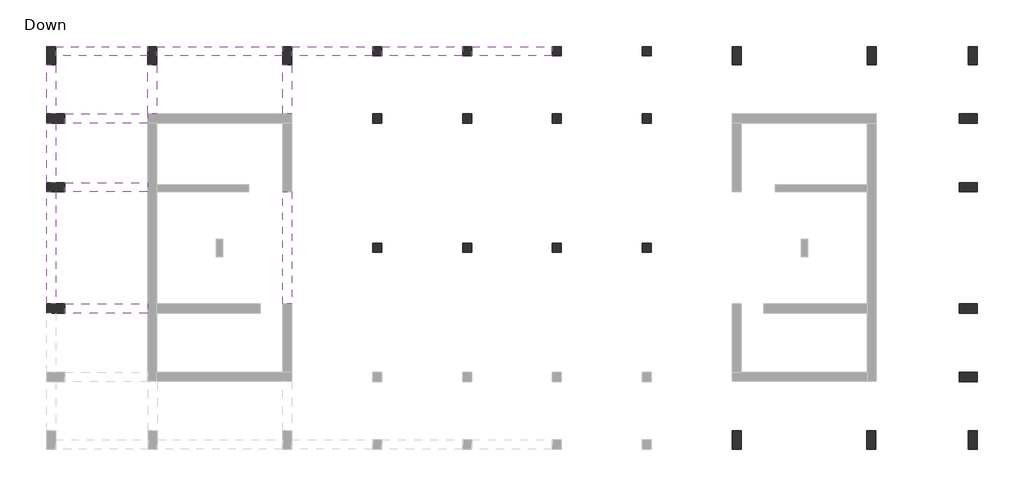
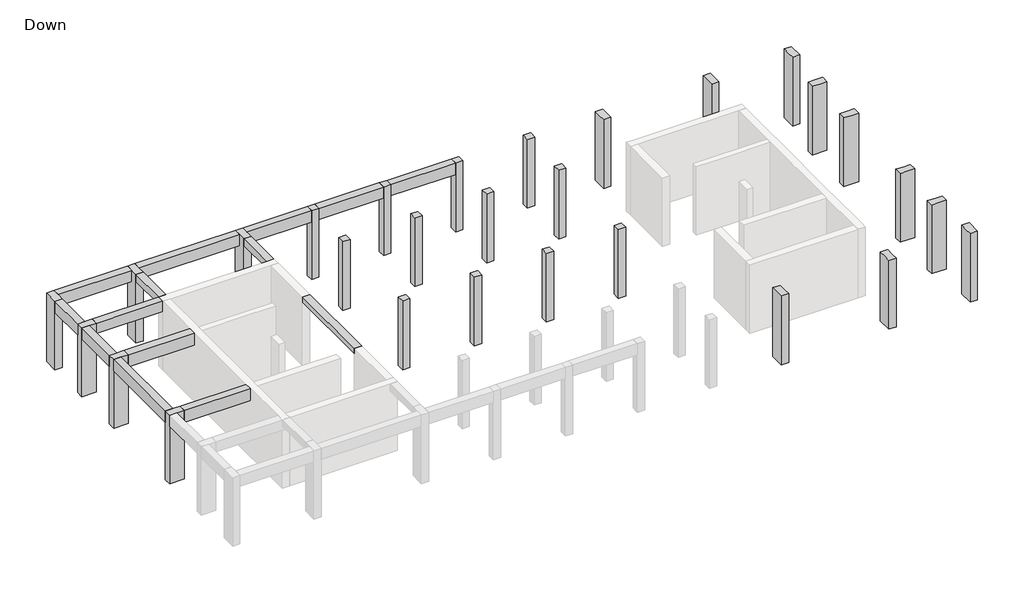
# One storey, part 2 of 2: 28 columns, 14 beams.
"""IFC4 building model written with IfcOpenShell, lengths in millimetres."""

from ifc_helpers import new_model, si_unit, frame, origin, place, context, project, spatial, polyline, outline, extrude, faceted_brep, element, save

model = new_model("IFC4")

# Units and contexts
model_context = context("Model", 3, world=origin())
ifc_project = project(units=[si_unit("LENGTHUNIT", "METRE", prefix="MILLI")], contexts=[model_context])

# Site, building, storey
site = spatial("IfcSite", under=ifc_project)
building = spatial("IfcBuilding", under=site)
storey = spatial("IfcBuildingStorey", under=building, Name="Down", Elevation=0.0)

# Beams
placement = place(None, origin())
element("IfcBeam", 1, ObjectType="Concrete Rectengular Beam : 40/30", at=placement, inside=storey, context=model_context, shape_type="SweptSolid", body=[
    extrude(outline(polyline([(-9870.3374688, 5392.831899), (-9470.3374688, 5392.831899), (-9470.3374688, 443.9061014), (-9870.3374688, 443.9061014), (-9870.3374688, 5392.831899)])), frame((0.0, 0.0, 3700.0), z_axis=(0.0, 0.0, 1.0), x_axis=(1.0, 0.0, 0.0)), (0.0, 0.0, 1.0), 300.0),
])
element("IfcBeam", 2, ObjectType="Concrete Rectengular Beam : 40/40", at=placement, inside=storey, context=model_context, shape_type="Brep", body=[
    faceted_brep([(-15412.8227448, 10981.7889465, 4000.0), (-15812.8227448, 10981.7889465, 4000.0), (-15812.8227448, 8813.6899891, 4000.0), (-15412.8227448, 8813.6899891, 4000.0), (-15812.8227448, 10981.7889465, 3600.0), (-15812.8227448, 8813.6899891, 3600.0), (-15812.8227448, 8813.6899891, 3850.0), (-15412.8227448, 10981.7889465, 3600.0), (-15412.8227448, 8813.6899891, 3600.0), (-15412.8227448, 8813.6899891, 3850.0)], [[[0, 1, 2, 3]], [[1, 4, 5, 6, 2]], [[4, 7, 8, 5]], [[7, 0, 3, 9, 8]], [[1, 0, 7, 4]], [[3, 2, 6, 5, 8, 9]]]),
])
element("IfcBeam", 3, ObjectType="Concrete Rectengular Beam : 40/40", at=placement, inside=storey, context=model_context, shape_type="Brep", body=[
    faceted_brep([(-9470.3374688, 10981.7889465, 4000.0), (-9870.3374688, 10981.7889465, 4000.0), (-9870.3374688, 8813.6899891, 4000.0), (-9470.3374688, 8813.6899891, 4000.0), (-9870.3374688, 10981.7889465, 3600.0), (-9870.3374688, 8813.6899891, 3600.0), (-9870.3374688, 8813.6899891, 3850.0), (-9470.3374688, 10981.7889465, 3600.0), (-9470.3374688, 8813.6899891, 3600.0)], [[[0, 1, 2, 3]], [[1, 4, 5, 6, 2]], [[4, 7, 8, 5]], [[7, 0, 3, 8]], [[1, 0, 7, 4]], [[3, 2, 6, 5, 8]]]),
])
element("IfcBeam", 4, ObjectType="Concrete Rectengular Beam : 40/60", at=placement, inside=storey, context=model_context, shape_type="Brep", body=[
    faceted_brep([(-19471.2573041, 8813.6899891, 4000.0), (-19471.2573041, 8413.6899891, 4000.0), (-15812.8227448, 8413.6899891, 4000.0), (-15812.8227448, 8813.6899891, 4000.0), (-19471.2573041, 8413.6899891, 3400.0), (-15812.8227448, 8413.6899891, 3400.0), (-15812.8227448, 8413.6899891, 3850.0), (-19471.2573041, 8813.6899891, 3400.0), (-15812.8227448, 8813.6899891, 3400.0), (-15812.8227448, 8813.6899891, 3850.0)], [[[0, 1, 2, 3]], [[1, 4, 5, 6, 2]], [[4, 7, 8, 5]], [[7, 0, 3, 9, 8]], [[1, 0, 7, 4]], [[3, 2, 6, 5, 8, 9]]]),
])
element("IfcBeam", 5, ObjectType="Concrete Rectengular Beam : 40/65", at=placement, inside=storey, context=model_context, shape_type="Brep", body=[
    faceted_brep([(-19871.2573041, 11781.7889465, 4000.0), (-19871.2573041, 11381.7889465, 4000.0), (-15812.8227448, 11381.7889465, 4000.0), (-15812.8227448, 11781.7889465, 4000.0), (-19871.2573041, 11781.7889465, 3350.0), (-15812.8227448, 11781.7889465, 3350.0), (-19871.2573041, 11381.7889465, 3350.0), (-15812.8227448, 11381.7889465, 3350.0), (-19871.2573041, 11381.7889465, 3850.0), (-15812.8227448, 11381.7889465, 3850.0)], [[[0, 1, 2, 3]], [[4, 0, 3, 5]], [[6, 4, 5, 7]], [[1, 8, 6, 7, 9, 2]], [[1, 0, 4, 6, 8]], [[3, 2, 9, 7, 5]]]),
])
element("IfcBeam", 6, ObjectType="Concrete Rectengular Beam : 40/65", at=placement, inside=storey, context=model_context, shape_type="Brep", body=[
    faceted_brep([(-15412.8227448, 11781.7889465, 4000.0), (-15412.8227448, 11381.7889465, 4000.0), (-9870.3374688, 11381.7889465, 4000.0), (-9870.3374688, 11781.7889465, 4000.0), (-15412.8227448, 11381.7889465, 3850.0), (-15412.8227448, 11381.7889465, 3350.0), (-9870.3374688, 11381.7889465, 3350.0), (-9870.3374688, 11381.7889465, 3850.0), (-15412.8227448, 11781.7889465, 3350.0), (-9870.3374688, 11781.7889465, 3350.0)], [[[0, 1, 2, 3]], [[1, 4, 5, 6, 7, 2]], [[5, 8, 9, 6]], [[8, 0, 3, 9]], [[1, 0, 8, 5, 4]], [[3, 2, 7, 6, 9]]]),
])
element("IfcBeam", 7, ObjectType="Concrete Rectengular Beam : 40/65", at=placement, inside=storey, context=model_context, shape_type="Brep", body=[
    faceted_brep([(-9470.3374688, 11781.7889465, 4000.0), (-9470.3374688, 11381.7889465, 4000.0), (-5908.6814696, 11381.7889465, 4000.0), (-5908.6814696, 11781.7889465, 4000.0), (-9470.3374688, 11381.7889465, 3770.0), (-9470.3374688, 11381.7889465, 3350.0), (-5908.6814696, 11381.7889465, 3350.0), (-9470.3374688, 11781.7889465, 3350.0), (-5908.6814696, 11781.7889465, 3350.0)], [[[0, 1, 2, 3]], [[1, 4, 5, 6, 2]], [[5, 7, 8, 6]], [[7, 0, 3, 8]], [[1, 0, 7, 5, 4]], [[3, 2, 6, 8]]]),
])
element("IfcBeam", 8, ObjectType="Concrete Rectengular Beam : 40/65", at=placement, inside=storey, context=model_context, shape_type="SweptSolid", body=[
    extrude(outline(polyline([(-5508.6814696, 11381.7889465), (-5508.6814696, 11781.7889465), (-1947.0254312, 11781.7889465), (-1947.0254312, 11381.7889465), (-5508.6814696, 11381.7889465)])), frame((0.0, 0.0, 3350.0), z_axis=(0.0, 0.0, 1.0), x_axis=(1.0, 0.0, 0.0)), (0.0, 0.0, 1.0), 650.0),
])
element("IfcBeam", 9, ObjectType="Concrete Rectengular Beam : 40/65", at=placement, inside=storey, context=model_context, shape_type="Brep", body=[
    faceted_brep([(-19871.2573041, 10981.7889465, 4000.0), (-20271.2573041, 10981.7889465, 4000.0), (-20271.2573041, 8813.6899891, 4000.0), (-19871.2573041, 8813.6899891, 4000.0), (-20271.2573041, 10981.7889465, 3350.0), (-20271.2573041, 8813.6899891, 3350.0), (-19871.2573041, 10981.7889465, 3350.0), (-19871.2573041, 8813.6899891, 3350.0), (-19871.2573041, 8813.6899891, 3850.0)], [[[0, 1, 2, 3]], [[1, 4, 5, 2]], [[4, 6, 7, 5]], [[6, 0, 3, 8, 7]], [[1, 0, 6, 4]], [[3, 2, 5, 7, 8]]]),
])
element("IfcBeam", 10, ObjectType="Concrete Rectengular Beam : 40/65", at=placement, inside=storey, context=model_context, shape_type="Brep", body=[
    faceted_brep([(-19871.2573041, 8413.6899891, 4000.0), (-20271.2573041, 8413.6899891, 4000.0), (-20271.2573041, 5788.9969998, 4000.0), (-19871.2573041, 5788.9969998, 4000.0), (-20271.2573041, 8413.6899891, 3350.0), (-20271.2573041, 5788.9969998, 3350.0), (-19871.2573041, 8413.6899891, 3350.0), (-19871.2573041, 5788.9969998, 3350.0), (-19871.2573041, 8413.6899891, 3850.0), (-19871.2573041, 5788.9969998, 3850.0)], [[[0, 1, 2, 3]], [[1, 4, 5, 2]], [[4, 6, 7, 5]], [[6, 8, 0, 3, 9, 7]], [[1, 0, 8, 6, 4]], [[3, 2, 5, 7, 9]]]),
])
element("IfcBeam", 11, ObjectType="Concrete Rectengular Beam : 40/65", at=placement, inside=storey, context=model_context, shape_type="Brep", body=[
    faceted_brep([(-19871.2573041, 5388.9969998, 4000.0), (-20271.2573041, 5388.9969998, 4000.0), (-20271.2573041, 443.9061014, 4000.0), (-19871.2573041, 443.9061014, 4000.0), (-20271.2573041, 5388.9969998, 3350.0), (-20271.2573041, 443.9061014, 3350.0), (-19871.2573041, 5388.9969998, 3350.0), (-19871.2573041, 443.9061014, 3350.0), (-19871.2573041, 5388.9969998, 3850.0), (-19871.2573041, 443.9061014, 3850.0)], [[[0, 1, 2, 3]], [[1, 4, 5, 2]], [[4, 6, 7, 5]], [[6, 8, 0, 3, 9, 7]], [[1, 0, 8, 6, 4]], [[3, 2, 5, 7, 9]]]),
])
element("IfcBeam", 12, ObjectType="Concrete Rectengular Beam : 40/65", at=placement, inside=storey, context=model_context, shape_type="SweptSolid", body=[
    extrude(outline(polyline([(-1547.0254312, 11381.7889465), (-1547.0254312, 11781.7889465), (2010.7993238, 11781.7889465), (2010.7993238, 11381.7889465), (-1547.0254312, 11381.7889465)])), frame((0.0, 0.0, 3350.0), z_axis=(0.0, 0.0, 1.0), x_axis=(1.0, 0.0, 0.0)), (0.0, 0.0, 1.0), 650.0),
])
element("IfcBeam", 13, ObjectType="Concrete Rectengular Beam : 40/70", at=placement, inside=storey, context=model_context, shape_type="Brep", body=[
    faceted_brep([(-19471.2573041, 443.9061014, 4000.0), (-19471.2573041, 43.9061014, 4000.0), (-15812.8227448, 43.9061014, 4000.0), (-15812.8227448, 443.9061014, 4000.0), (-19471.2573041, 43.9061014, 3300.0), (-15812.8227448, 43.9061014, 3300.0), (-15812.8227448, 43.9061014, 3850.0), (-19471.2573041, 443.9061014, 3300.0), (-15812.8227448, 443.9061014, 3300.0), (-15812.8227448, 443.9061014, 3850.0)], [[[0, 1, 2, 3]], [[1, 4, 5, 6, 2]], [[4, 7, 8, 5]], [[7, 0, 3, 9, 8]], [[1, 0, 7, 4]], [[3, 2, 6, 5, 8, 9]]]),
])
element("IfcBeam", 14, ObjectType="Concrete Rectengular Beam : 40/70", at=placement, inside=storey, context=model_context, shape_type="Brep", body=[
    faceted_brep([(-19471.2573041, 5788.9969998, 4000.0), (-19471.2573041, 5388.9969998, 4000.0), (-15812.8227448, 5388.9969998, 4000.0), (-15812.8227448, 5788.9969998, 4000.0), (-19471.2573041, 5388.9969998, 3300.0), (-15812.8227448, 5388.9969998, 3300.0), (-15812.8227448, 5388.9969998, 3850.0), (-19471.2573041, 5788.9969998, 3300.0), (-15812.8227448, 5788.9969998, 3300.0), (-15812.8227448, 5788.9969998, 3850.0)], [[[0, 1, 2, 3]], [[1, 4, 5, 6, 2]], [[4, 7, 8, 5]], [[7, 0, 3, 9, 8]], [[1, 0, 7, 4]], [[3, 2, 6, 5, 8, 9]]]),
])

# Columns
element("IfcColumn", 15, ObjectType="Concrete Rectengular Column : 40/40", at=placement, inside=storey, context=model_context, shape_type="Brep", body=[
    faceted_brep([(-5508.6814696, 8813.6899891, 0.0), (-5508.6814696, 8413.6899891, 0.0), (-5908.6814696, 8413.6899891, 0.0), (-5908.6814696, 8813.6899891, 0.0), (-5508.6814696, 8813.6899891, 4000.0), (-5508.6814696, 8413.6899891, 4000.0), (-5508.6814696, 8413.6899891, 3770.0), (-5508.6814696, 8813.6899891, 3770.0), (-5908.6814696, 8413.6899891, 4000.0), (-5908.6814696, 8413.6899891, 3770.0), (-5908.6814696, 8813.6899891, 4000.0), (-5908.6814696, 8813.6899891, 3770.0)], [[[0, 1, 2, 3]], [[4, 5, 6, 1, 0, 7]], [[5, 8, 9, 2, 1, 6]], [[8, 10, 11, 3, 2, 9]], [[10, 4, 7, 0, 3, 11]], [[4, 10, 8, 5]]]),
])
element("IfcColumn", 16, ObjectType="Concrete Rectengular Column : 40/40", at=placement, inside=storey, context=model_context, shape_type="Brep", body=[
    faceted_brep([(-1547.0254312, 8813.6899891, 0.0), (-1547.0254312, 8413.6899891, 0.0), (-1947.0254312, 8413.6899891, 0.0), (-1947.0254312, 8813.6899891, 0.0), (-1547.0254312, 8813.6899891, 4000.0), (-1547.0254312, 8413.6899891, 4000.0), (-1547.0254312, 8413.6899891, 3770.0), (-1547.0254312, 8813.6899891, 3770.0), (-1947.0254312, 8413.6899891, 4000.0), (-1947.0254312, 8413.6899891, 3770.0), (-1947.0254312, 8813.6899891, 4000.0), (-1947.0254312, 8813.6899891, 3770.0)], [[[0, 1, 2, 3]], [[4, 5, 6, 1, 0, 7]], [[5, 8, 9, 2, 1, 6]], [[8, 10, 11, 3, 2, 9]], [[10, 4, 7, 0, 3, 11]], [[4, 10, 8, 5]]]),
])
element("IfcColumn", 17, ObjectType="Concrete Rectengular Column : 40/40", at=placement, inside=storey, context=model_context, shape_type="Brep", body=[
    faceted_brep([(-1547.0254312, 3116.4509414, 0.0), (-1547.0254312, 2716.4509414, 0.0), (-1947.0254312, 2716.4509414, 0.0), (-1947.0254312, 3116.4509414, 0.0), (-1547.0254312, 3116.4509414, 4000.0), (-1547.0254312, 2716.4509414, 4000.0), (-1547.0254312, 2716.4509414, 3770.0), (-1547.0254312, 3116.4509414, 3770.0), (-1947.0254312, 2716.4509414, 4000.0), (-1947.0254312, 2716.4509414, 3770.0), (-1947.0254312, 3116.4509414, 4000.0), (-1947.0254312, 3116.4509414, 3770.0)], [[[0, 1, 2, 3]], [[4, 5, 6, 1, 0, 7]], [[5, 8, 9, 2, 1, 6]], [[8, 10, 11, 3, 2, 9]], [[10, 4, 7, 0, 3, 11]], [[4, 10, 8, 5]]]),
])
element("IfcColumn", 18, ObjectType="Concrete Rectengular Column : 40/40", at=placement, inside=storey, context=model_context, shape_type="Brep", body=[
    faceted_brep([(-5508.6814696, 3116.4509414, 0.0), (-5508.6814696, 2716.4509414, 0.0), (-5908.6814696, 2716.4509414, 0.0), (-5908.6814696, 3116.4509414, 0.0), (-5508.6814696, 3116.4509414, 4000.0), (-5508.6814696, 2716.4509414, 4000.0), (-5508.6814696, 2716.4509414, 3770.0), (-5508.6814696, 3116.4509414, 3770.0), (-5908.6814696, 2716.4509414, 4000.0), (-5908.6814696, 2716.4509414, 3770.0), (-5908.6814696, 3116.4509414, 4000.0), (-5908.6814696, 3116.4509414, 3770.0)], [[[0, 1, 2, 3]], [[4, 5, 6, 1, 0, 7]], [[5, 8, 9, 2, 1, 6]], [[8, 10, 11, 3, 2, 9]], [[10, 4, 7, 0, 3, 11]], [[4, 10, 8, 5]]]),
])
element("IfcColumn", 19, ObjectType="Concrete Rectengular Column : 40/40", at=placement, inside=storey, context=model_context, shape_type="Brep", body=[
    faceted_brep([(-5508.6814696, 11781.7889465, 0.0), (-5508.6814696, 11381.7889465, 0.0), (-5908.6814696, 11381.7889465, 0.0), (-5908.6814696, 11781.7889465, 0.0), (-5508.6814696, 11781.7889465, 4000.0), (-5508.6814696, 11381.7889465, 4000.0), (-5508.6814696, 11381.7889465, 3350.0), (-5508.6814696, 11781.7889465, 3350.0), (-5908.6814696, 11381.7889465, 4000.0), (-5908.6814696, 11381.7889465, 3350.0), (-5908.6814696, 11781.7889465, 4000.0), (-5908.6814696, 11781.7889465, 3350.0)], [[[0, 1, 2, 3]], [[4, 5, 6, 1, 0, 7]], [[5, 8, 9, 2, 1, 6]], [[8, 10, 11, 3, 2, 9]], [[10, 4, 7, 0, 3, 11]], [[4, 10, 8, 5]]]),
])
element("IfcColumn", 20, ObjectType="Concrete Rectengular Column : 40/40", at=placement, inside=storey, context=model_context, shape_type="Brep", body=[
    faceted_brep([(-1547.0254312, 11781.7889465, 0.0), (-1547.0254312, 11381.7889465, 0.0), (-1947.0254312, 11381.7889465, 0.0), (-1947.0254312, 11781.7889465, 0.0), (-1547.0254312, 11781.7889465, 4000.0), (-1547.0254312, 11381.7889465, 4000.0), (-1947.0254312, 11381.7889465, 4000.0), (-1947.0254312, 11381.7889465, 3350.0), (-1947.0254312, 11781.7889465, 4000.0), (-1947.0254312, 11781.7889465, 3350.0)], [[[0, 1, 2, 3]], [[4, 5, 1, 0]], [[5, 6, 7, 2, 1]], [[6, 8, 9, 3, 2, 7]], [[8, 4, 0, 3, 9]], [[4, 8, 6, 5]]]),
])
element("IfcColumn", 21, ObjectType="Concrete Rectengular Column : 40/40", at=placement, inside=storey, context=model_context, shape_type="Brep", body=[
    faceted_brep([(5972.4553623, 8813.6899891, 0.0), (6372.4553623, 8813.6899891, 0.0), (6372.4553623, 8413.6899891, 0.0), (5972.4553623, 8413.6899891, 0.0), (5972.4553623, 8813.6899891, 4000.0), (5972.4553623, 8813.6899891, 3770.0), (5972.4553623, 8413.6899891, 3770.0), (5972.4553623, 8413.6899891, 4000.0), (6372.4553623, 8413.6899891, 3770.0), (6372.4553623, 8413.6899891, 4000.0), (6372.4553623, 8813.6899891, 3770.0), (6372.4553623, 8813.6899891, 4000.0)], [[[0, 1, 2, 3]], [[4, 5, 0, 3, 6, 7]], [[7, 6, 3, 2, 8, 9]], [[9, 8, 2, 1, 10, 11]], [[11, 10, 1, 0, 5, 4]], [[4, 7, 9, 11]]]),
])
element("IfcColumn", 22, ObjectType="Concrete Rectengular Column : 40/40", at=placement, inside=storey, context=model_context, shape_type="Brep", body=[
    faceted_brep([(2010.7993238, 8813.6899891, 0.0), (2410.7993238, 8813.6899891, 0.0), (2410.7993238, 8413.6899891, 0.0), (2010.7993238, 8413.6899891, 0.0), (2010.7993238, 8813.6899891, 4000.0), (2010.7993238, 8813.6899891, 3770.0), (2010.7993238, 8413.6899891, 3770.0), (2010.7993238, 8413.6899891, 4000.0), (2410.7993238, 8413.6899891, 3770.0), (2410.7993238, 8413.6899891, 4000.0), (2410.7993238, 8813.6899891, 3770.0), (2410.7993238, 8813.6899891, 4000.0)], [[[0, 1, 2, 3]], [[4, 5, 0, 3, 6, 7]], [[7, 6, 3, 2, 8, 9]], [[9, 8, 2, 1, 10, 11]], [[11, 10, 1, 0, 5, 4]], [[4, 7, 9, 11]]]),
])
element("IfcColumn", 23, ObjectType="Concrete Rectengular Column : 40/40", at=placement, inside=storey, context=model_context, shape_type="Brep", body=[
    faceted_brep([(2010.7993238, 3116.4509414, 0.0), (2410.7993238, 3116.4509414, 0.0), (2410.7993238, 2716.4509414, 0.0), (2010.7993238, 2716.4509414, 0.0), (2010.7993238, 3116.4509414, 4000.0), (2010.7993238, 3116.4509414, 3770.0), (2010.7993238, 2716.4509414, 3770.0), (2010.7993238, 2716.4509414, 4000.0), (2410.7993238, 2716.4509414, 3770.0), (2410.7993238, 2716.4509414, 4000.0), (2410.7993238, 3116.4509414, 3770.0), (2410.7993238, 3116.4509414, 4000.0)], [[[0, 1, 2, 3]], [[4, 5, 0, 3, 6, 7]], [[7, 6, 3, 2, 8, 9]], [[9, 8, 2, 1, 10, 11]], [[11, 10, 1, 0, 5, 4]], [[4, 7, 9, 11]]]),
])
element("IfcColumn", 24, ObjectType="Concrete Rectengular Column : 40/40", at=placement, inside=storey, context=model_context, shape_type="Brep", body=[
    faceted_brep([(5972.4553623, 3116.4509414, 0.0), (6372.4553623, 3116.4509414, 0.0), (6372.4553623, 2716.4509414, 0.0), (5972.4553623, 2716.4509414, 0.0), (5972.4553623, 3116.4509414, 4000.0), (5972.4553623, 3116.4509414, 3770.0), (5972.4553623, 2716.4509414, 3770.0), (5972.4553623, 2716.4509414, 4000.0), (6372.4553623, 2716.4509414, 3770.0), (6372.4553623, 2716.4509414, 4000.0), (6372.4553623, 3116.4509414, 3770.0), (6372.4553623, 3116.4509414, 4000.0)], [[[0, 1, 2, 3]], [[4, 5, 0, 3, 6, 7]], [[7, 6, 3, 2, 8, 9]], [[9, 8, 2, 1, 10, 11]], [[11, 10, 1, 0, 5, 4]], [[4, 7, 9, 11]]]),
])
element("IfcColumn", 25, ObjectType="Concrete Rectengular Column : 40/40", at=placement, inside=storey, context=model_context, shape_type="Brep", body=[
    faceted_brep([(5972.4553623, 11781.7889465, 0.0), (6372.4553623, 11781.7889465, 0.0), (6372.4553623, 11381.7889465, 0.0), (5972.4553623, 11381.7889465, 0.0), (5972.4553623, 11781.7889465, 4000.0), (5972.4553623, 11781.7889465, 3350.0), (5972.4553623, 11381.7889465, 3350.0), (5972.4553623, 11381.7889465, 4000.0), (6372.4553623, 11381.7889465, 3350.0), (6372.4553623, 11381.7889465, 4000.0), (6372.4553623, 11781.7889465, 3350.0), (6372.4553623, 11781.7889465, 4000.0)], [[[0, 1, 2, 3]], [[4, 5, 0, 3, 6, 7]], [[7, 6, 3, 2, 8, 9]], [[9, 8, 2, 1, 10, 11]], [[11, 10, 1, 0, 5, 4]], [[4, 7, 9, 11]]]),
])
element("IfcColumn", 26, ObjectType="Concrete Rectengular Column : 40/40", at=placement, inside=storey, context=model_context, shape_type="Brep", body=[
    faceted_brep([(2010.7993238, 11781.7889465, 0.0), (2410.7993238, 11781.7889465, 0.0), (2410.7993238, 11381.7889465, 0.0), (2010.7993238, 11381.7889465, 0.0), (2010.7993238, 11781.7889465, 4000.0), (2010.7993238, 11381.7889465, 4000.0), (2410.7993238, 11381.7889465, 3350.0), (2410.7993238, 11381.7889465, 4000.0), (2410.7993238, 11781.7889465, 3350.0), (2410.7993238, 11781.7889465, 4000.0)], [[[0, 1, 2, 3]], [[4, 0, 3, 5]], [[5, 3, 2, 6, 7]], [[7, 6, 2, 1, 8, 9]], [[9, 8, 1, 0, 4]], [[4, 5, 7, 9]]]),
])
element("IfcColumn", 27, ObjectType="Concrete Rectengular Column : 40/80", at=placement, inside=storey, context=model_context, shape_type="Brep", body=[
    faceted_brep([(-19871.2573041, 11781.7889465, 0.0), (-19871.2573041, 10981.7889465, 0.0), (-20271.2573041, 10981.7889465, 0.0), (-20271.2573041, 11781.7889465, 0.0), (-19871.2573041, 11781.7889465, 4000.0), (-19871.2573041, 11381.7889465, 4000.0), (-19871.2573041, 10981.7889465, 4000.0), (-20271.2573041, 10981.7889465, 4000.0), (-20271.2573041, 11781.7889465, 4000.0)], [[[0, 1, 2, 3]], [[4, 5, 6, 1, 0]], [[6, 7, 2, 1]], [[7, 8, 3, 2]], [[8, 4, 0, 3]], [[4, 8, 7, 6, 5]]]),
])
element("IfcColumn", 28, ObjectType="Concrete Rectengular Column : 40/80", at=placement, inside=storey, context=model_context, shape_type="Brep", body=[
    faceted_brep([(-20271.2573041, 8813.6899891, 0.0), (-19471.2573041, 8813.6899891, 0.0), (-19471.2573041, 8413.6899891, 0.0), (-20271.2573041, 8413.6899891, 0.0), (-20271.2573041, 8813.6899891, 4000.0), (-19871.2573041, 8813.6899891, 4000.0), (-19471.2573041, 8813.6899891, 4000.0), (-19471.2573041, 8413.6899891, 4000.0), (-19871.2573041, 8413.6899891, 4000.0), (-20271.2573041, 8413.6899891, 4000.0)], [[[0, 1, 2, 3]], [[4, 5, 6, 1, 0]], [[6, 7, 2, 1]], [[7, 8, 9, 3, 2]], [[9, 4, 0, 3]], [[4, 9, 8, 7, 6, 5]]]),
])
element("IfcColumn", 29, ObjectType="Concrete Rectengular Column : 40/80", at=placement, inside=storey, context=model_context, shape_type="Brep", body=[
    faceted_brep([(-20271.2573041, 5788.9969998, 0.0), (-19471.2573041, 5788.9969998, 0.0), (-19471.2573041, 5388.9969998, 0.0), (-20271.2573041, 5388.9969998, 0.0), (-20271.2573041, 5788.9969998, 4000.0), (-19871.2573041, 5788.9969998, 4000.0), (-19471.2573041, 5788.9969998, 4000.0), (-19471.2573041, 5388.9969998, 4000.0), (-19871.2573041, 5388.9969998, 4000.0), (-20271.2573041, 5388.9969998, 4000.0)], [[[0, 1, 2, 3]], [[4, 5, 6, 1, 0]], [[6, 7, 2, 1]], [[7, 8, 9, 3, 2]], [[9, 4, 0, 3]], [[4, 9, 8, 7, 6, 5]]]),
])
element("IfcColumn", 30, ObjectType="Concrete Rectengular Column : 40/80", at=placement, inside=storey, context=model_context, shape_type="Brep", body=[
    faceted_brep([(-20271.2573041, 443.9061014, 0.0), (-19471.2573041, 443.9061014, 0.0), (-19471.2573041, 43.9061014, 0.0), (-20271.2573041, 43.9061014, 0.0), (-20271.2573041, 443.9061014, 4000.0), (-19871.2573041, 443.9061014, 4000.0), (-19471.2573041, 443.9061014, 4000.0), (-19471.2573041, 43.9061014, 4000.0), (-19871.2573041, 43.9061014, 4000.0), (-20271.2573041, 43.9061014, 4000.0)], [[[0, 1, 2, 3]], [[4, 5, 6, 1, 0]], [[6, 7, 2, 1]], [[7, 8, 9, 3, 2]], [[9, 4, 0, 3]], [[4, 9, 8, 7, 6, 5]]]),
])
element("IfcColumn", 31, ObjectType="Concrete Rectengular Column : 40/80", at=placement, inside=storey, context=model_context, shape_type="Brep", body=[
    faceted_brep([(-15412.8227448, 11781.7889465, 0.0), (-15412.8227448, 10981.7889465, 0.0), (-15812.8227448, 10981.7889465, 0.0), (-15812.8227448, 11781.7889465, 0.0), (-15412.8227448, 11781.7889465, 4000.0), (-15412.8227448, 11381.7889465, 4000.0), (-15412.8227448, 10981.7889465, 4000.0), (-15812.8227448, 10981.7889465, 4000.0), (-15812.8227448, 11381.7889465, 4000.0), (-15812.8227448, 11781.7889465, 4000.0)], [[[0, 1, 2, 3]], [[4, 5, 6, 1, 0]], [[6, 7, 2, 1]], [[7, 8, 9, 3, 2]], [[9, 4, 0, 3]], [[4, 9, 8, 7, 6, 5]]]),
])
element("IfcColumn", 32, ObjectType="Concrete Rectengular Column : 40/80", at=placement, inside=storey, context=model_context, shape_type="Brep", body=[
    faceted_brep([(-9470.3374688, 11781.7889465, 0.0), (-9470.3374688, 10981.7889465, 0.0), (-9870.3374688, 10981.7889465, 0.0), (-9870.3374688, 11781.7889465, 0.0), (-9470.3374688, 11781.7889465, 4000.0), (-9470.3374688, 11381.7889465, 4000.0), (-9470.3374688, 10981.7889465, 4000.0), (-9870.3374688, 10981.7889465, 4000.0), (-9870.3374688, 11381.7889465, 4000.0), (-9870.3374688, 11781.7889465, 4000.0)], [[[0, 1, 2, 3]], [[4, 5, 6, 1, 0]], [[6, 7, 2, 1]], [[7, 8, 9, 3, 2]], [[9, 4, 0, 3]], [[4, 9, 8, 7, 6, 5]]]),
])
element("IfcColumn", 33, ObjectType="Concrete Rectengular Column : 40/80", at=placement, inside=storey, context=model_context, shape_type="Brep", body=[
    faceted_brep([(20335.0311968, 11781.7889465, 0.0), (20735.0311968, 11781.7889465, 0.0), (20735.0311968, 10981.7889465, 0.0), (20335.0311968, 10981.7889465, 0.0), (20335.0311968, 11781.7889465, 4000.0), (20335.0311968, 10981.7889465, 4000.0), (20335.0311968, 11381.7889465, 4000.0), (20735.0311968, 10981.7889465, 4000.0), (20735.0311968, 11781.7889465, 4000.0)], [[[0, 1, 2, 3]], [[4, 0, 3, 5, 6]], [[5, 3, 2, 7]], [[7, 2, 1, 8]], [[8, 1, 0, 4]], [[4, 6, 5, 7, 8]]]),
])
element("IfcColumn", 34, ObjectType="Concrete Rectengular Column : 40/80", at=placement, inside=storey, context=model_context, shape_type="Brep", body=[
    faceted_brep([(20735.0311968, 8813.6899891, 0.0), (20735.0311968, 8413.6899891, 0.0), (19935.0311968, 8413.6899891, 0.0), (19935.0311968, 8813.6899891, 0.0), (20735.0311968, 8813.6899891, 4000.0), (19935.0311968, 8813.6899891, 4000.0), (20335.0311968, 8813.6899891, 4000.0), (19935.0311968, 8413.6899891, 4000.0), (20735.0311968, 8413.6899891, 4000.0), (20335.0311968, 8413.6899891, 4000.0)], [[[0, 1, 2, 3]], [[4, 0, 3, 5, 6]], [[5, 3, 2, 7]], [[7, 2, 1, 8, 9]], [[8, 1, 0, 4]], [[4, 6, 5, 7, 9, 8]]]),
])
element("IfcColumn", 35, ObjectType="Concrete Rectengular Column : 40/80", at=placement, inside=storey, context=model_context, shape_type="Brep", body=[
    faceted_brep([(20735.0311968, 5788.9969998, 0.0), (20735.0311968, 5388.9969998, 0.0), (19935.0311968, 5388.9969998, 0.0), (19935.0311968, 5788.9969998, 0.0), (20735.0311968, 5788.9969998, 4000.0), (19935.0311968, 5788.9969998, 4000.0), (20335.0311968, 5788.9969998, 4000.0), (19935.0311968, 5388.9969998, 4000.0), (20735.0311968, 5388.9969998, 4000.0), (20335.0311968, 5388.9969998, 4000.0)], [[[0, 1, 2, 3]], [[4, 0, 3, 5, 6]], [[5, 3, 2, 7]], [[7, 2, 1, 8, 9]], [[8, 1, 0, 4]], [[4, 6, 5, 7, 9, 8]]]),
])
element("IfcColumn", 36, ObjectType="Concrete Rectengular Column : 40/80", at=placement, inside=storey, context=model_context, shape_type="Brep", body=[
    faceted_brep([(20735.0311968, 443.9061014, 0.0), (20735.0311968, 43.9061014, 0.0), (19935.0311968, 43.9061014, 0.0), (19935.0311968, 443.9061014, 0.0), (20735.0311968, 443.9061014, 4000.0), (19935.0311968, 443.9061014, 4000.0), (20335.0311968, 443.9061014, 4000.0), (19935.0311968, 43.9061014, 4000.0), (20735.0311968, 43.9061014, 4000.0), (20335.0311968, 43.9061014, 4000.0)], [[[0, 1, 2, 3]], [[4, 0, 3, 5, 6]], [[5, 3, 2, 7]], [[7, 2, 1, 8, 9]], [[8, 1, 0, 4]], [[4, 6, 5, 7, 9, 8]]]),
])
element("IfcColumn", 37, ObjectType="Concrete Rectengular Column : 40/80", at=placement, inside=storey, context=model_context, shape_type="Brep", body=[
    faceted_brep([(20735.0311968, -2574.5007845, 0.0), (20735.0311968, -2974.5007845, 0.0), (19935.0311968, -2974.5007845, 0.0), (19935.0311968, -2574.5007845, 0.0), (20735.0311968, -2574.5007845, 4000.0), (19935.0311968, -2574.5007845, 4000.0), (20335.0311968, -2574.5007845, 4000.0), (19935.0311968, -2974.5007845, 4000.0), (20735.0311968, -2974.5007845, 4000.0), (20335.0311968, -2974.5007845, 4000.0)], [[[0, 1, 2, 3]], [[4, 0, 3, 5, 6]], [[5, 3, 2, 7]], [[7, 2, 1, 8, 9]], [[8, 1, 0, 4]], [[4, 6, 5, 7, 9, 8]]]),
])
element("IfcColumn", 38, ObjectType="Concrete Rectengular Column : 40/80", at=placement, inside=storey, context=model_context, shape_type="Brep", body=[
    faceted_brep([(20335.0311968, -5152.7195656, 0.0), (20735.0311968, -5152.7195656, 0.0), (20735.0311968, -5952.7195656, 0.0), (20335.0311968, -5952.7195656, 0.0), (20335.0311968, -5152.7195656, 4000.0), (20335.0311968, -5952.7195656, 4000.0), (20335.0311968, -5548.8870638, 4000.0), (20735.0311968, -5952.7195656, 4000.0), (20735.0311968, -5152.7195656, 4000.0)], [[[0, 1, 2, 3]], [[4, 0, 3, 5, 6]], [[5, 3, 2, 7]], [[7, 2, 1, 8]], [[8, 1, 0, 4]], [[4, 6, 5, 7, 8]]]),
])
element("IfcColumn", 39, ObjectType="Concrete Rectengular Column : 40/80", at=placement, inside=storey, context=model_context, shape_type="Brep", body=[
    faceted_brep([(15855.0311968, -5152.7195656, 0.0), (16255.0311968, -5152.7195656, 0.0), (16255.0311968, -5952.7195656, 0.0), (15855.0311968, -5952.7195656, 0.0), (15855.0311968, -5152.7195656, 4000.0), (15855.0311968, -5952.7195656, 4000.0), (15855.0311968, -5548.8870638, 4000.0), (16255.0311968, -5952.7195656, 4000.0), (16255.0311968, -5152.7195656, 4000.0), (16255.0311968, -5548.8870638, 4000.0)], [[[0, 1, 2, 3]], [[4, 0, 3, 5, 6]], [[5, 3, 2, 7]], [[7, 2, 1, 8, 9]], [[8, 1, 0, 4]], [[4, 6, 5, 7, 9, 8]]]),
])
element("IfcColumn", 40, ObjectType="Concrete Rectengular Column : 40/80", at=placement, inside=storey, context=model_context, shape_type="Brep", body=[
    faceted_brep([(9934.1113614, -5152.7195656, 0.0), (10334.1113614, -5152.7195656, 0.0), (10334.1113614, -5952.7195656, 0.0), (9934.1113614, -5952.7195656, 0.0), (9934.1113614, -5152.7195656, 4000.0), (9934.1113614, -5952.7195656, 4000.0), (9934.1113614, -5548.8870638, 4000.0), (10334.1113614, -5952.7195656, 4000.0), (10334.1113614, -5152.7195656, 4000.0), (10334.1113614, -5548.8870638, 4000.0)], [[[0, 1, 2, 3]], [[4, 0, 3, 5, 6]], [[5, 3, 2, 7]], [[7, 2, 1, 8, 9]], [[8, 1, 0, 4]], [[4, 6, 5, 7, 9, 8]]]),
])
element("IfcColumn", 41, ObjectType="Concrete Rectengular Column : 40/80", at=placement, inside=storey, context=model_context, shape_type="Brep", body=[
    faceted_brep([(15876.5966375, 11781.7889465, 0.0), (16276.5966375, 11781.7889465, 0.0), (16276.5966375, 10981.7889465, 0.0), (15876.5966375, 10981.7889465, 0.0), (15876.5966375, 11781.7889465, 4000.0), (15876.5966375, 10981.7889465, 4000.0), (15876.5966375, 11381.7889465, 4000.0), (16276.5966375, 10981.7889465, 4000.0), (16276.5966375, 11781.7889465, 4000.0), (16276.5966375, 11381.7889465, 4000.0)], [[[0, 1, 2, 3]], [[4, 0, 3, 5, 6]], [[5, 3, 2, 7]], [[7, 2, 1, 8, 9]], [[8, 1, 0, 4]], [[4, 6, 5, 7, 9, 8]]]),
])
element("IfcColumn", 42, ObjectType="Concrete Rectengular Column : 40/80", at=placement, inside=storey, context=model_context, shape_type="Brep", body=[
    faceted_brep([(9934.1113614, 11781.7889465, 0.0), (10334.1113614, 11781.7889465, 0.0), (10334.1113614, 10981.7889465, 0.0), (9934.1113614, 10981.7889465, 0.0), (9934.1113614, 11781.7889465, 4000.0), (9934.1113614, 10981.7889465, 4000.0), (9934.1113614, 11381.7889465, 4000.0), (10334.1113614, 10981.7889465, 4000.0), (10334.1113614, 11781.7889465, 4000.0), (10334.1113614, 11381.7889465, 4000.0)], [[[0, 1, 2, 3]], [[4, 0, 3, 5, 6]], [[5, 3, 2, 7]], [[7, 2, 1, 8, 9]], [[8, 1, 0, 4]], [[4, 6, 5, 7, 9, 8]]]),
])

save(model, "model.ifc")

# Revit data of these elements
# Type "Concrete Rectengular Beam : 40/30"
#   Length [instance default] = 152.4 cm
#   b = 40 cm
#   h = 30 cm
#   Structural Material [instance default] = Concrete
#   Assembly Code = ""
# Type "Concrete Rectengular Beam : 40/40"
#   Length [instance default] = 152.4 cm
#   b = 40 cm
#   h = 40 cm
#   Structural Material [instance default] = Concrete
#   Assembly Code = ""
# Type "Concrete Rectengular Beam : 40/60"
#   Length [instance default] = 152.4 cm
#   b = 40 cm
#   h = 60 cm
#   Structural Material [instance default] = Concrete
#   Assembly Code = ""
# Type "Concrete Rectengular Beam : 40/65"
#   Length [instance default] = 152.4 cm
#   b = 40 cm
#   h = 65 cm
#   Structural Material [instance default] = Concrete
#   Assembly Code = ""
# Type "Concrete Rectengular Beam : 40/70"
#   Length [instance default] = 152.4 cm
#   b = 40 cm
#   h = 70 cm
#   Structural Material [instance default] = Concrete
#   Assembly Code = ""
# Type "Concrete Rectengular Column : 40/40"
#   b = 40 cm
#   h = 40 cm
#   Structural Material [instance default] = Concrete
# Type "Concrete Rectengular Column : 40/80"
#   b = 40 cm
#   h = 80 cm
#   Structural Material [instance default] = Concrete
# Element 1 (IfcBeam, "Concrete Rectengular Beam : 40/30")
#   Comments = ""
#   Mark = "B1"
#   SOFiSTiK_AMG_Comments = ""
#   SOFiSTiK_AMG_Scheduled = yes
#   SOFiSTiK_AMG_Adjusted = yes
#   Structural Material = Concrete
#   Phase Created = New Construction
#   Materials on its faces: "Concrete"
# Element 2 (IfcBeam, "Concrete Rectengular Beam : 40/40")
#   Comments = ""
#   Mark = "B5"
#   SOFiSTiK_AMG_Comments = ""
#   SOFiSTiK_AMG_Scheduled = yes
#   SOFiSTiK_AMG_Adjusted = yes
#   Structural Material = Concrete
#   Phase Created = New Construction
#   Materials on its faces: "Concrete"
# Element 3 (IfcBeam, "Concrete Rectengular Beam : 40/40")
#   Comments = ""
#   Mark = "B6"
#   SOFiSTiK_AMG_Comments = ""
#   SOFiSTiK_AMG_Scheduled = yes
#   SOFiSTiK_AMG_Adjusted = yes
#   Structural Material = Concrete
#   Phase Created = New Construction
#   Materials on its faces: "Concrete"
# Element 4 (IfcBeam, "Concrete Rectengular Beam : 40/60")
#   Comments = ""
#   Mark = "B11"
#   SOFiSTiK_AMG_Comments = ""
#   SOFiSTiK_AMG_Scheduled = yes
#   SOFiSTiK_AMG_Adjusted = yes
#   Structural Material = Concrete
#   Phase Created = New Construction
#   Materials on its faces: "Concrete"
# Element 5 (IfcBeam, "Concrete Rectengular Beam : 40/65")
#   Comments = ""
#   Mark = "B15"
#   SOFiSTiK_AMG_Comments = ""
#   SOFiSTiK_AMG_Scheduled = yes
#   SOFiSTiK_AMG_Adjusted = yes
#   Structural Material = Concrete
#   Phase Created = New Construction
#   Materials on its faces: "Concrete"
# Element 6 (IfcBeam, "Concrete Rectengular Beam : 40/65")
#   Comments = ""
#   Mark = "B16"
#   SOFiSTiK_AMG_Comments = ""
#   SOFiSTiK_AMG_Scheduled = yes
#   SOFiSTiK_AMG_Adjusted = yes
#   Structural Material = Concrete
#   Phase Created = New Construction
#   Materials on its faces: "Concrete"
# Element 7 (IfcBeam, "Concrete Rectengular Beam : 40/65")
#   Comments = ""
#   Mark = "B19"
#   SOFiSTiK_AMG_Comments = ""
#   SOFiSTiK_AMG_Scheduled = yes
#   SOFiSTiK_AMG_Adjusted = yes
#   Structural Material = Concrete
#   Phase Created = New Construction
#   Materials on its faces: "Concrete"
# Element 8 (IfcBeam, "Concrete Rectengular Beam : 40/65")
#   Comments = ""
#   Mark = "B20"
#   SOFiSTiK_AMG_Comments = ""
#   SOFiSTiK_AMG_Scheduled = yes
#   SOFiSTiK_AMG_Adjusted = yes
#   Structural Material = Concrete
#   Phase Created = New Construction
#   Materials on its faces: "Concrete"
# Element 9 (IfcBeam, "Concrete Rectengular Beam : 40/65")
#   Comments = ""
#   Mark = "B23"
#   SOFiSTiK_AMG_Comments = ""
#   SOFiSTiK_AMG_Scheduled = yes
#   SOFiSTiK_AMG_Adjusted = yes
#   Structural Material = Concrete
#   Phase Created = New Construction
#   Materials on its faces: "Concrete"
# Element 10 (IfcBeam, "Concrete Rectengular Beam : 40/65")
#   Comments = ""
#   Mark = "B24"
#   SOFiSTiK_AMG_Comments = ""
#   SOFiSTiK_AMG_Scheduled = yes
#   SOFiSTiK_AMG_Adjusted = yes
#   Structural Material = Concrete
#   Phase Created = New Construction
#   Materials on its faces: "Concrete"
# Element 11 (IfcBeam, "Concrete Rectengular Beam : 40/65")
#   Comments = ""
#   Mark = "B25"
#   SOFiSTiK_AMG_Comments = ""
#   SOFiSTiK_AMG_Scheduled = yes
#   SOFiSTiK_AMG_Adjusted = yes
#   Structural Material = Concrete
#   Phase Created = New Construction
#   Materials on its faces: "Concrete"
# Element 12 (IfcBeam, "Concrete Rectengular Beam : 40/65")
#   Comments = ""
#   Mark = "B41"
#   SOFiSTiK_AMG_Comments = ""
#   SOFiSTiK_AMG_Scheduled = yes
#   SOFiSTiK_AMG_Adjusted = yes
#   Structural Material = Concrete
#   Phase Created = New Construction
#   Materials on its faces: "Concrete"
# Element 13 (IfcBeam, "Concrete Rectengular Beam : 40/70")
#   Comments = ""
#   Mark = "B43"
#   SOFiSTiK_AMG_Comments = ""
#   SOFiSTiK_AMG_Scheduled = yes
#   SOFiSTiK_AMG_Adjusted = yes
#   Structural Material = Concrete
#   Phase Created = New Construction
#   Materials on its faces: "Concrete"
# Element 14 (IfcBeam, "Concrete Rectengular Beam : 40/70")
#   Comments = ""
#   Mark = "B44"
#   SOFiSTiK_AMG_Comments = ""
#   SOFiSTiK_AMG_Scheduled = yes
#   SOFiSTiK_AMG_Adjusted = yes
#   Structural Material = Concrete
#   Phase Created = New Construction
#   Materials on its faces: "Concrete"
# Element 15 (IfcColumn, "Concrete Rectengular Column : 40/40")
#   Comments = ""
#   Mark = "C1"
#   SOFiSTiK_AMG_Comments = ""
#   SOFiSTiK_AMG_Scheduled = yes
#   SOFiSTiK_AMG_Adjusted = yes
#   Structural Material = Concrete
#   Phase Created = New Construction
#   Materials on its faces: "Concrete"
# Element 16 (IfcColumn, "Concrete Rectengular Column : 40/40")
#   Comments = ""
#   Mark = "C2"
#   SOFiSTiK_AMG_Comments = ""
#   SOFiSTiK_AMG_Scheduled = yes
#   SOFiSTiK_AMG_Adjusted = yes
#   Structural Material = Concrete
#   Phase Created = New Construction
#   Materials on its faces: "Concrete"
# Element 17 (IfcColumn, "Concrete Rectengular Column : 40/40")
#   Comments = ""
#   Mark = "C3"
#   SOFiSTiK_AMG_Comments = ""
#   SOFiSTiK_AMG_Scheduled = yes
#   SOFiSTiK_AMG_Adjusted = yes
#   Structural Material = Concrete
#   Phase Created = New Construction
#   Materials on its faces: "Concrete"
# Element 18 (IfcColumn, "Concrete Rectengular Column : 40/40")
#   Comments = ""
#   Mark = "C4"
#   SOFiSTiK_AMG_Comments = ""
#   SOFiSTiK_AMG_Scheduled = yes
#   SOFiSTiK_AMG_Adjusted = yes
#   Structural Material = Concrete
#   Phase Created = New Construction
#   Materials on its faces: "Concrete"
# Element 19 (IfcColumn, "Concrete Rectengular Column : 40/40")
#   Comments = ""
#   Mark = "C9"
#   SOFiSTiK_AMG_Comments = ""
#   SOFiSTiK_AMG_Scheduled = yes
#   SOFiSTiK_AMG_Adjusted = yes
#   Structural Material = Concrete
#   Phase Created = New Construction
#   Materials on its faces: "Concrete"
# Element 20 (IfcColumn, "Concrete Rectengular Column : 40/40")
#   Comments = ""
#   Mark = "C10"
#   SOFiSTiK_AMG_Comments = ""
#   SOFiSTiK_AMG_Scheduled = yes
#   SOFiSTiK_AMG_Adjusted = yes
#   Structural Material = Concrete
#   Phase Created = New Construction
#   Materials on its faces: "Concrete"
# Element 21 (IfcColumn, "Concrete Rectengular Column : 40/40")
#   Comments = ""
#   Mark = "C11"
#   SOFiSTiK_AMG_Comments = ""
#   SOFiSTiK_AMG_Scheduled = yes
#   SOFiSTiK_AMG_Adjusted = yes
#   Structural Material = Concrete
#   Phase Created = New Construction
#   Materials on its faces: "Concrete"
# Element 22 (IfcColumn, "Concrete Rectengular Column : 40/40")
#   Comments = ""
#   Mark = "C12"
#   SOFiSTiK_AMG_Comments = ""
#   SOFiSTiK_AMG_Scheduled = yes
#   SOFiSTiK_AMG_Adjusted = yes
#   Structural Material = Concrete
#   Phase Created = New Construction
#   Materials on its faces: "Concrete"
# Element 23 (IfcColumn, "Concrete Rectengular Column : 40/40")
#   Comments = ""
#   Mark = "C13"
#   SOFiSTiK_AMG_Comments = ""
#   SOFiSTiK_AMG_Scheduled = yes
#   SOFiSTiK_AMG_Adjusted = yes
#   Structural Material = Concrete
#   Phase Created = New Construction
#   Materials on its faces: "Concrete"
# Element 24 (IfcColumn, "Concrete Rectengular Column : 40/40")
#   Comments = ""
#   Mark = "C14"
#   SOFiSTiK_AMG_Comments = ""
#   SOFiSTiK_AMG_Scheduled = yes
#   SOFiSTiK_AMG_Adjusted = yes
#   Structural Material = Concrete
#   Phase Created = New Construction
#   Materials on its faces: "Concrete"
# Element 25 (IfcColumn, "Concrete Rectengular Column : 40/40")
#   Comments = ""
#   Mark = "C19"
#   SOFiSTiK_AMG_Comments = ""
#   SOFiSTiK_AMG_Scheduled = yes
#   SOFiSTiK_AMG_Adjusted = yes
#   Structural Material = Concrete
#   Phase Created = New Construction
#   Materials on its faces: "Concrete"
# Element 26 (IfcColumn, "Concrete Rectengular Column : 40/40")
#   Comments = ""
#   Mark = "C20"
#   SOFiSTiK_AMG_Comments = ""
#   SOFiSTiK_AMG_Scheduled = yes
#   SOFiSTiK_AMG_Adjusted = yes
#   Structural Material = Concrete
#   Phase Created = New Construction
#   Materials on its faces: "Concrete"
# Element 27 (IfcColumn, "Concrete Rectengular Column : 40/80")
#   Comments = ""
#   Mark = "C21"
#   SOFiSTiK_AMG_Comments = ""
#   SOFiSTiK_AMG_Scheduled = yes
#   SOFiSTiK_AMG_Adjusted = yes
#   Structural Material = Concrete
#   Phase Created = New Construction
#   Materials on its faces: "Concrete"
# Element 28 (IfcColumn, "Concrete Rectengular Column : 40/80")
#   Comments = ""
#   Mark = "C22"
#   SOFiSTiK_AMG_Comments = ""
#   SOFiSTiK_AMG_Scheduled = yes
#   SOFiSTiK_AMG_Adjusted = yes
#   Structural Material = Concrete
#   Phase Created = New Construction
#   Materials on its faces: "Concrete"
# Element 29 (IfcColumn, "Concrete Rectengular Column : 40/80")
#   Comments = ""
#   Mark = "C23"
#   SOFiSTiK_AMG_Comments = ""
#   SOFiSTiK_AMG_Scheduled = yes
#   SOFiSTiK_AMG_Adjusted = yes
#   Structural Material = Concrete
#   Phase Created = New Construction
#   Materials on its faces: "Concrete"
# Element 30 (IfcColumn, "Concrete Rectengular Column : 40/80")
#   Comments = ""
#   Mark = "C24"
#   SOFiSTiK_AMG_Comments = ""
#   SOFiSTiK_AMG_Scheduled = yes
#   SOFiSTiK_AMG_Adjusted = yes
#   Structural Material = Concrete
#   Phase Created = New Construction
#   Materials on its faces: "Concrete"
# Element 31 (IfcColumn, "Concrete Rectengular Column : 40/80")
#   Comments = ""
#   Mark = "C29"
#   SOFiSTiK_AMG_Comments = ""
#   SOFiSTiK_AMG_Scheduled = yes
#   SOFiSTiK_AMG_Adjusted = yes
#   Structural Material = Concrete
#   Phase Created = New Construction
#   Materials on its faces: "Concrete"
# Element 32 (IfcColumn, "Concrete Rectengular Column : 40/80")
#   Comments = ""
#   Mark = "C30"
#   SOFiSTiK_AMG_Comments = ""
#   SOFiSTiK_AMG_Scheduled = yes
#   SOFiSTiK_AMG_Adjusted = yes
#   Structural Material = Concrete
#   Phase Created = New Construction
#   Materials on its faces: "Concrete"
# Element 33 (IfcColumn, "Concrete Rectengular Column : 40/80")
#   Comments = ""
#   Mark = "C31"
#   SOFiSTiK_AMG_Comments = ""
#   SOFiSTiK_AMG_Scheduled = yes
#   SOFiSTiK_AMG_Adjusted = yes
#   Structural Material = Concrete
#   Phase Created = New Construction
#   Materials on its faces: "Concrete"
# Element 34 (IfcColumn, "Concrete Rectengular Column : 40/80")
#   Comments = ""
#   Mark = "C32"
#   SOFiSTiK_AMG_Comments = ""
#   SOFiSTiK_AMG_Scheduled = yes
#   SOFiSTiK_AMG_Adjusted = yes
#   Structural Material = Concrete
#   Phase Created = New Construction
#   Materials on its faces: "Concrete"
# Element 35 (IfcColumn, "Concrete Rectengular Column : 40/80")
#   Comments = ""
#   Mark = "C33"
#   SOFiSTiK_AMG_Comments = ""
#   SOFiSTiK_AMG_Scheduled = yes
#   SOFiSTiK_AMG_Adjusted = yes
#   Structural Material = Concrete
#   Phase Created = New Construction
#   Materials on its faces: "Concrete"
# Element 36 (IfcColumn, "Concrete Rectengular Column : 40/80")
#   Comments = ""
#   Mark = "C34"
#   SOFiSTiK_AMG_Comments = ""
#   SOFiSTiK_AMG_Scheduled = yes
#   SOFiSTiK_AMG_Adjusted = yes
#   Structural Material = Concrete
#   Phase Created = New Construction
#   Materials on its faces: "Concrete"
# Element 37 (IfcColumn, "Concrete Rectengular Column : 40/80")
#   Comments = ""
#   Mark = "C35"
#   SOFiSTiK_AMG_Comments = ""
#   SOFiSTiK_AMG_Scheduled = yes
#   SOFiSTiK_AMG_Adjusted = yes
#   Structural Material = Concrete
#   Phase Created = New Construction
#   Materials on its faces: "Concrete"
# Element 38 (IfcColumn, "Concrete Rectengular Column : 40/80")
#   Comments = ""
#   Mark = "C36"
#   SOFiSTiK_AMG_Comments = ""
#   SOFiSTiK_AMG_Scheduled = yes
#   SOFiSTiK_AMG_Adjusted = yes
#   Structural Material = Concrete
#   Phase Created = New Construction
#   Materials on its faces: "Concrete"
# Element 39 (IfcColumn, "Concrete Rectengular Column : 40/80")
#   Comments = ""
#   Mark = "C37"
#   SOFiSTiK_AMG_Comments = ""
#   SOFiSTiK_AMG_Scheduled = yes
#   SOFiSTiK_AMG_Adjusted = yes
#   Structural Material = Concrete
#   Phase Created = New Construction
#   Materials on its faces: "Concrete"
# Element 40 (IfcColumn, "Concrete Rectengular Column : 40/80")
#   Comments = ""
#   Mark = "C38"
#   SOFiSTiK_AMG_Comments = ""
#   SOFiSTiK_AMG_Scheduled = yes
#   SOFiSTiK_AMG_Adjusted = yes
#   Structural Material = Concrete
#   Phase Created = New Construction
#   Materials on its faces: "Concrete"
# Element 41 (IfcColumn, "Concrete Rectengular Column : 40/80")
#   Comments = ""
#   Mark = "C39"
#   SOFiSTiK_AMG_Comments = ""
#   SOFiSTiK_AMG_Scheduled = yes
#   SOFiSTiK_AMG_Adjusted = yes
#   Structural Material = Concrete
#   Phase Created = New Construction
#   Materials on its faces: "Concrete"
# Element 42 (IfcColumn, "Concrete Rectengular Column : 40/80")
#   Comments = ""
#   Mark = "C40"
#   SOFiSTiK_AMG_Comments = ""
#   SOFiSTiK_AMG_Scheduled = yes
#   SOFiSTiK_AMG_Adjusted = yes
#   Structural Material = Concrete
#   Phase Created = New Construction
#   Materials on its faces: "Concrete"
# Materials
#   "Concrete": class "Concrete", colour RGB 192 192 192, transparency 0, Keynote = "01000", Description = "Cast-in-place concrete", Cost = 0
